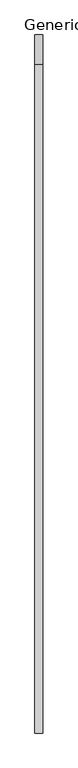
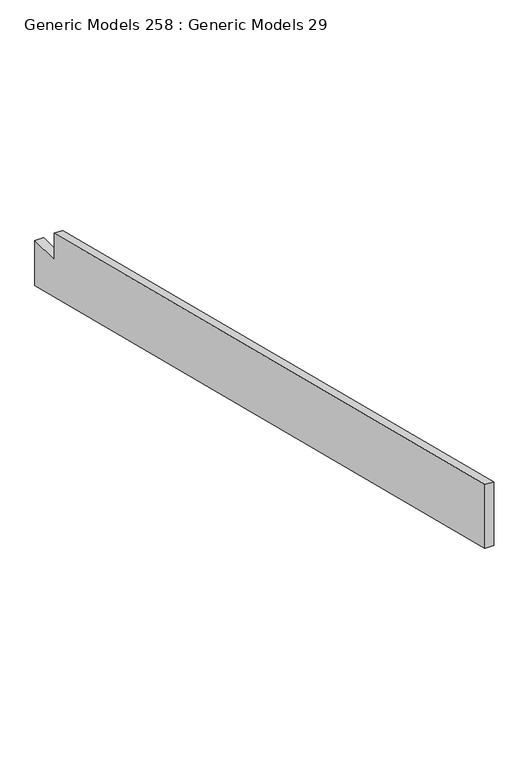
"""IFC4 building model written with IfcOpenShell, lengths in millimetres: proxy geometry, Generic Models 258 : Generic Models 29."""

from ifc_helpers import new_model, si_unit, frame, origin, place, context, project, spatial, polyline, outline, extrude, source, transform, mapped, element, save


def generic_models_258_generic_models_29_e6fa0126(model_context):
    return source(origin(), model_context, "Body", "SweptSolid", [
        extrude(outline(polyline([(12591.4769662, 129267.4777207), (9187.8769662, 130118.3777207), (9187.8769662, 130412.9220789), (12445.4269662, 129598.5345789), (12445.4269662, 129476.4447278), (12591.4769662, 129476.4447278), (12591.4769662, 129267.4777207)])), frame((1065.7410488, 0.0, 0.0), z_axis=(1.0, 0.0, 0.0), x_axis=(0.0, 1.0, 0.0)), (0.0, 0.0, 1.0), 38.1),
    ])


if __name__ == "__main__":
    model = new_model("IFC4")
    model_context = context("Model", 3, world=origin())
    ifc_project = project(units=[si_unit("LENGTHUNIT", "METRE", prefix="MILLI")], contexts=[model_context])
    site = spatial("IfcSite", under=ifc_project)
    building = spatial("IfcBuilding", under=site)
    placement = place(None, origin())
    generic_models_258_generic_models_29_shape = generic_models_258_generic_models_29_e6fa0126(model_context)
    element("IfcBuildingElementProxy", 1, Name="Generic Models 258 : Generic Models 29", ObjectType="Generic Models 258 : Generic Models 29", at=placement, inside=building, context=model_context, shape_type="MappedRepresentation", body=[
        mapped(generic_models_258_generic_models_29_shape, transform((0.0, 0.0, 0.0), x_axis=(1.0, 0.0, 0.0), y_axis=(0.0, 1.0, 0.0), z_axis=(0.0, 0.0, 1.0))),
    ])
    save(model, "model.ifc")

# Revit data of these elements
# Element 1 (IfcBuildingElementProxy, "Generic Models 258 : Generic Models 29")
#   Materials on its faces: "_STRUCTURAL MEMBER (SEE STRUCT. DWGS)"
# Materials
#   "_STRUCTURAL MEMBER (SEE STRUCT. DWGS)": class "Generic", colour RGB 209 182 141, transparency 0, Cost = 0
